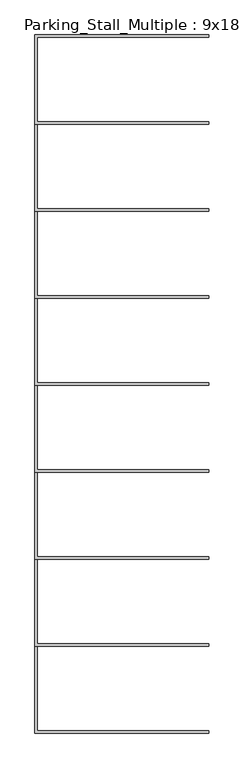
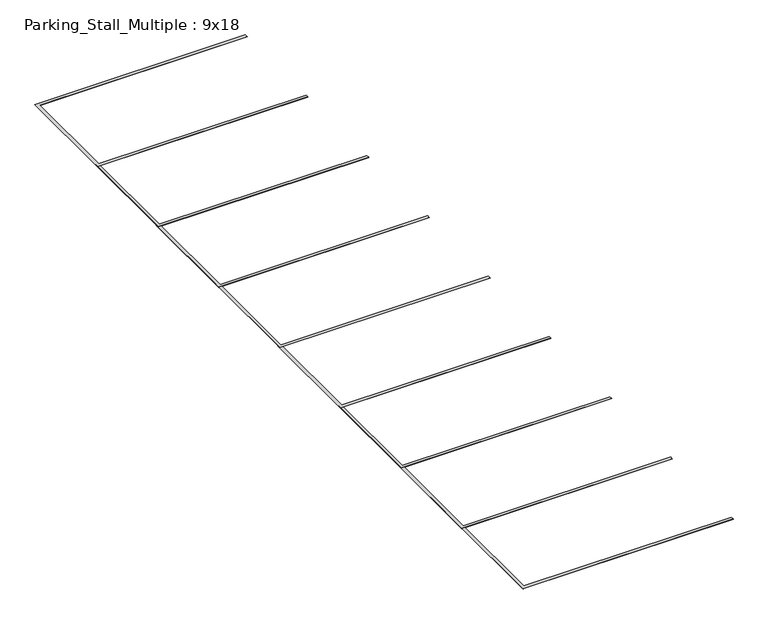
"""IFC4 building model written with IfcOpenShell, lengths in millimetres: proxy geometry, Parking_Stall_Multiple : 9x18."""

import ifcopenshell
import ifcopenshell.guid

model = None  # the IFC model being written
_history = None  # IfcOwnerHistory: only IFC2X3 demands one
_inside = {}  # id of a spatial element -> (the spatial element, [elements in it])
_under = {}  # id of a project, library or spatial element -> (it, [spatial elements below it])
_declared = {}  # id of a project -> (the project, [libraries it declares])
_typed = {}  # id of a type object -> (the type object, [elements of that type])
_made_of = {}  # id of a material, layer set ... -> (it, [elements and type objects made of it])


def new_model(schema):
    """Start an empty IFC model of exactly this schema.

    Asked for "IFC4X3", IfcOpenShell would pick the latest addendum, in which some entities
    have other attributes; the version numbers below select the first issue.
    IFC2X3 requires an IfcOwnerHistory on every rooted entity: one is made here for all.
    """
    global model, _history
    if schema == "IFC4X3":
        model = ifcopenshell.file(schema_version=(4, 3, 0, 0))
    else:
        model = ifcopenshell.file(schema=schema)
    _inside.clear()
    _under.clear()
    _declared.clear()
    _typed.clear()
    _made_of.clear()
    _history = None
    if model.schema == "IFC2X3":
        org = make("IfcOrganization", Name="unknown")
        user = make(
            "IfcPersonAndOrganization",
            ThePerson=make("IfcPerson", FamilyName="unknown"),
            TheOrganization=org,
        )
        app = make(
            "IfcApplication",
            ApplicationDeveloper=org,
            Version="unknown",
            ApplicationFullName="unknown",
            ApplicationIdentifier="unknown",
        )
        _history = make(
            "IfcOwnerHistory",
            OwningUser=user,
            OwningApplication=app,
            ChangeAction="ADDED",
            CreationDate=0,
        )
    return model


def make(cls, **values):
    """One entity of the class cls with the attributes given. An attribute that is None is left unset."""
    return model.create_entity(
        cls, **{name: value for name, value in values.items() if value is not None}
    )


def rooted(cls, **values):
    """An entity with a GlobalId (a new one), such as an element, a storey or a relation."""
    return make(cls, GlobalId=ifcopenshell.guid.new(), OwnerHistory=_history, **values)


def si_unit(unit_type, name, prefix=None):
    """IfcSIUnit, for example si_unit("LENGTHUNIT", "METRE", prefix="MILLI")."""
    return make("IfcSIUnit", UnitType=unit_type, Prefix=prefix, Name=name)


def assignment(units):
    """IfcUnitAssignment: the units of a project."""
    return None if units is None else make("IfcUnitAssignment", Units=units)


def point(xyz):
    """IfcCartesianPoint."""
    return None if xyz is None else make("IfcCartesianPoint", Coordinates=xyz)


def direction(xyz):
    """IfcDirection."""
    return None if xyz is None else make("IfcDirection", DirectionRatios=xyz)


def frame(location, z_axis=None, x_axis=None):
    """IfcAxis2Placement3D, a coordinate frame: its origin and axes. An axis left out is left unset."""
    return make(
        "IfcAxis2Placement3D",
        Location=point(location),
        Axis=direction(z_axis),
        RefDirection=direction(x_axis),
    )


def origin():
    """The frame at (0, 0, 0) with its axes left unset."""
    return frame((0.0, 0.0, 0.0))


def origin_with_axes():
    """The frame at (0, 0, 0) with the z axis (0, 0, 1) and the x axis (1, 0, 0) written out."""
    return frame((0.0, 0.0, 0.0), z_axis=(0.0, 0.0, 1.0), x_axis=(1.0, 0.0, 0.0))


def place(relative_to, where):
    """IfcLocalPlacement: puts the frame where relative to a parent placement (None: the world)."""
    return make(
        "IfcLocalPlacement", PlacementRelTo=relative_to, RelativePlacement=where
    )


def context(
    kind, dimensions, precision=None, world=None, true_north=None, identifier=None
):
    """IfcGeometricRepresentationContext, for example the 3D "Model" context."""
    return make(
        "IfcGeometricRepresentationContext",
        ContextIdentifier=identifier,
        ContextType=kind,
        CoordinateSpaceDimension=dimensions,
        Precision=precision,
        WorldCoordinateSystem=world,
        TrueNorth=true_north,
    )


def project(units=None, contexts=None):
    """IfcProject with its units and contexts."""
    return rooted(
        "IfcProject",
        Name="project",
        RepresentationContexts=contexts,
        UnitsInContext=assignment(units),
    )


def spatial(cls, under=None, at=None, **own):
    """A site, building, storey or space (cls), placed at a placement, below another one or the project."""
    s = rooted(cls, ObjectPlacement=at, **own)
    if under is not None:
        _under.setdefault(under.id(), (under, []))[1].append(s)
    return s


def polyline(points):
    """IfcPolyline through the points."""
    return make("IfcPolyline", Points=[point(p) for p in points])


def outline(outer, holes=None, kind="AREA"):
    """IfcArbitraryClosedProfileDef: a profile drawn as a closed curve; with holes, ...WithVoids."""
    if holes is None:
        return make("IfcArbitraryClosedProfileDef", ProfileType=kind, OuterCurve=outer)
    return make(
        "IfcArbitraryProfileDefWithVoids",
        ProfileType=kind,
        OuterCurve=outer,
        InnerCurves=holes,
    )


def extrude(swept, where, along, depth):
    """IfcExtrudedAreaSolid: the profile swept, set in the frame where, extruded along a direction by depth."""
    return make(
        "IfcExtrudedAreaSolid",
        SweptArea=swept,
        Position=where,
        ExtrudedDirection=direction(along),
        Depth=depth,
    )


def shape(context_of_items, identifier, shape_type, items):
    """IfcShapeRepresentation: the items that make up one representation, for example the "Body"."""
    return make(
        "IfcShapeRepresentation",
        ContextOfItems=context_of_items,
        RepresentationIdentifier=identifier,
        RepresentationType=shape_type,
        Items=items,
    )


def source(mapping_origin, context_of_items, identifier, shape_type, items):
    """IfcRepresentationMap: a shape defined once, which mapped items show again and again."""
    return make(
        "IfcRepresentationMap",
        MappingOrigin=mapping_origin,
        MappedRepresentation=shape(context_of_items, identifier, shape_type, items),
    )


def transform(
    local_origin,
    x_axis=None,
    y_axis=None,
    z_axis=None,
    scale=None,
    scale2=None,
    scale3=None,
    uniform=True,
):
    """IfcCartesianTransformationOperator3D, or its non-uniform kind. x_axis, y_axis, z_axis: its Axis1, 2, 3."""
    if uniform:
        return make(
            "IfcCartesianTransformationOperator3D",
            Axis1=direction(x_axis),
            Axis2=direction(y_axis),
            LocalOrigin=point(local_origin),
            Scale=scale,
            Axis3=direction(z_axis),
        )
    return make(
        "IfcCartesianTransformationOperator3DnonUniform",
        Axis1=direction(x_axis),
        Axis2=direction(y_axis),
        LocalOrigin=point(local_origin),
        Scale=scale,
        Axis3=direction(z_axis),
        Scale2=scale2,
        Scale3=scale3,
    )


def mapped(mapping_source, mapping_target):
    """IfcMappedItem: shows the shape of a source again, moved by a transform."""
    return make(
        "IfcMappedItem", MappingSource=mapping_source, MappingTarget=mapping_target
    )


def made_of(thing, what):
    """Note that an element or type object is made of a material, layer set ...; save() writes the relation."""
    if what is not None:
        _made_of.setdefault(what.id(), (what, []))[1].append(thing)
    return thing


def element(
    cls,
    number,
    at=None,
    inside=None,
    cuts=None,
    type_object=None,
    material=None,
    context=None,
    identifier="Body",
    shape_type=None,
    held_by="IfcProductDefinitionShape",
    body=None,
    shapes=None,
    **own,
):
    """One element of the class cls, such as IfcWall. Its Tag is "e" and its number.

    at: its placement. inside: the storey or other place that contains it. cuts: it is an
    opening in that element (IfcRelVoidsElement). A single representation is given by context,
    identifier, shape_type and body (its items); several are given by shapes. held_by: the class
    of the entity that holds the representations. save() writes the other relations.
    """
    e = rooted(cls, Tag="e%d" % number, ObjectPlacement=at, **own)
    if body is not None:
        shapes = [shape(context, identifier, shape_type, body)]
    if shapes is not None:
        e.Representation = make(held_by, Representations=shapes)
    if inside is not None:
        _inside.setdefault(inside.id(), (inside, []))[1].append(e)
    if cuts is not None:
        rooted(
            "IfcRelVoidsElement", RelatingBuildingElement=cuts, RelatedOpeningElement=e
        )
    if type_object is not None:
        _typed.setdefault(type_object.id(), (type_object, []))[1].append(e)
    return made_of(e, material)


def aggregate(whole, parts):
    """IfcRelAggregates: a whole, such as a stair, and the parts it consists of."""
    return rooted("IfcRelAggregates", RelatingObject=whole, RelatedObjects=parts)


def save(model, path):
    """Write the relations noted so far, then the file.

    IfcRelAggregates (storeys below a building ...), IfcRelContainedInSpatialStructure (elements
    in a storey), IfcRelDefinesByType, IfcRelAssociatesMaterial and IfcRelDeclares: one each for
    every whole, place, type object, material and project.
    """
    for whole, parts in _under.values():
        aggregate(whole, parts)
    for where, things in _inside.values():
        rooted(
            "IfcRelContainedInSpatialStructure",
            RelatedElements=things,
            RelatingStructure=where,
        )
    for kind, things in _typed.values():
        rooted("IfcRelDefinesByType", RelatedObjects=things, RelatingType=kind)
    for what, things in _made_of.values():
        rooted("IfcRelAssociatesMaterial", RelatedObjects=things, RelatingMaterial=what)
    for by, libraries in _declared.values():
        rooted("IfcRelDeclares", RelatingContext=by, RelatedDefinitions=libraries)
    model.write(path)


def parking_stall_multiple_9x18_41294f2a(model_context):
    return source(origin(), model_context, "Body", "SweptSolid", [
        extrude(outline(polyline([(5486.4, 19202.4), (0.0, 19202.4), (0.0, 22021.8), (5486.4, 22021.8), (5486.4, 21945.6), (76.2, 21945.6), (76.2, 19278.6), (5486.4, 19278.6), (5486.4, 19202.4)])), origin_with_axes(), (0.0, 0.0, 1.0), 6.35),
        extrude(outline(polyline([(5486.4, 16459.2), (0.0, 16459.2), (0.0, 19278.6), (5486.4, 19278.6), (5486.4, 19202.4), (76.2, 19202.4), (76.2, 16535.4), (5486.4, 16535.4), (5486.4, 16459.2)])), origin_with_axes(), (0.0, 0.0, 1.0), 6.35),
        extrude(outline(polyline([(5486.4, 13716.0), (0.0, 13716.0), (0.0, 16535.4), (5486.4, 16535.4), (5486.4, 16459.2), (76.2, 16459.2), (76.2, 13792.2), (5486.4, 13792.2), (5486.4, 13716.0)])), origin_with_axes(), (0.0, 0.0, 1.0), 6.35),
        extrude(outline(polyline([(5486.4, 10972.8), (0.0, 10972.8), (0.0, 13792.2), (5486.4, 13792.2), (5486.4, 13716.0), (76.2, 13716.0), (76.2, 11049.0), (5486.4, 11049.0), (5486.4, 10972.8)])), origin_with_axes(), (0.0, 0.0, 1.0), 6.35),
        extrude(outline(polyline([(5486.4, 8229.6), (0.0, 8229.6), (0.0, 11049.0), (5486.4, 11049.0), (5486.4, 10972.8), (76.2, 10972.8), (76.2, 8305.8), (5486.4, 8305.8), (5486.4, 8229.6)])), origin_with_axes(), (0.0, 0.0, 1.0), 6.35),
        extrude(outline(polyline([(5486.4, 5486.4), (0.0, 5486.4), (0.0, 8305.8), (5486.4, 8305.8), (5486.4, 8229.6), (76.2, 8229.6), (76.2, 5562.6), (5486.4, 5562.6), (5486.4, 5486.4)])), origin_with_axes(), (0.0, 0.0, 1.0), 6.35),
        extrude(outline(polyline([(5486.4, 2743.2), (0.0, 2743.2), (0.0, 5562.6), (5486.4, 5562.6), (5486.4, 5486.4), (76.2, 5486.4), (76.2, 2819.4), (5486.4, 2819.4), (5486.4, 2743.2)])), origin_with_axes(), (0.0, 0.0, 1.0), 6.35),
        extrude(outline(polyline([(5486.4, 0.0), (0.0, 0.0), (0.0, 2819.4), (5486.4, 2819.4), (5486.4, 2743.2), (76.2, 2743.2), (76.2, 76.2), (5486.4, 76.2), (5486.4, 0.0)])), origin_with_axes(), (0.0, 0.0, 1.0), 6.35),
    ])


if __name__ == "__main__":
    model = new_model("IFC4")
    model_context = context("Model", 3, world=origin())
    ifc_project = project(units=[si_unit("LENGTHUNIT", "METRE", prefix="MILLI")], contexts=[model_context])
    site = spatial("IfcSite", under=ifc_project)
    building = spatial("IfcBuilding", under=site)
    placement = place(None, origin())
    parking_stall_multiple_9x18_shape = parking_stall_multiple_9x18_41294f2a(model_context)
    element("IfcBuildingElementProxy", 1, Name="Parking_Stall_Multiple : 9x18", ObjectType="Parking_Stall_Multiple : 9x18", at=placement, inside=building, context=model_context, shape_type="MappedRepresentation", body=[
        mapped(parking_stall_multiple_9x18_shape, transform((0.0, 0.0, 0.0), x_axis=(1.0, 0.0, 0.0), y_axis=(0.0, 1.0, 0.0), z_axis=(0.0, 0.0, 1.0))),
    ])
    save(model, "model.ifc")

# Revit data of these elements
# Type "Parking_Stall_Multiple : 9x18"
#   Parking_Width_M = 9' - 0"
#   Parking_Run_Length [instance default] = 65' - 0"
#   Parking_Line_Width = 0' - 3"
#   Parking_Length_M = 18' - 0"
#   Single_Parking_Visibility [instance default] = no
#   Parking_ADA_Symbol = no
#   ParkingUnitsArray [instance default] = 7
#   ParkingUnits [instance default] = 7
#   Multiple_Parking_Visibility [instance default] = yes
#   Parking_Line_Material = none
# Element 1 (IfcBuildingElementProxy, "Parking_Stall_Multiple : 9x18")
#   Parking_Run_Length = 70' - 11.05727"
#   ParkingUnitsArray = 8
#   ParkingUnits = 8
